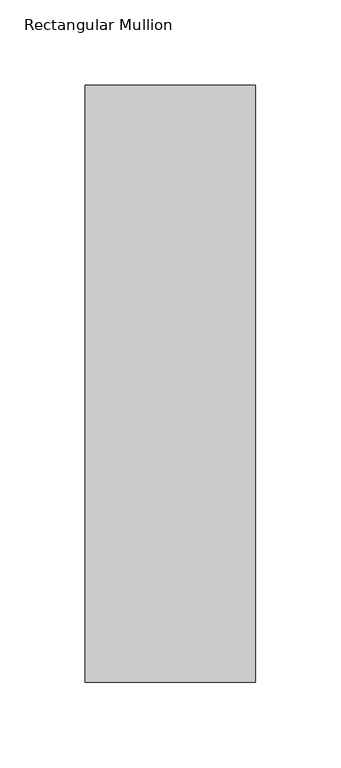
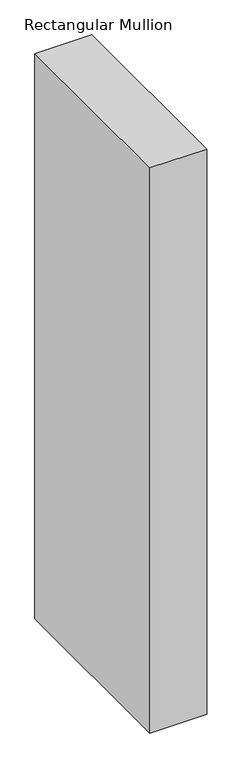
"""IFC4 building model written with IfcOpenShell, lengths in millimetres: member geometry, Rectangular Mullion : WWm-100x350-100mmOffset."""

from ifc_helpers import new_model, si_unit, frame, origin, place, context, project, spatial, polyline, outline, extrude, source, transform, mapped, element, save


def rectangular_mullion_53cec424(model_context):
    return source(origin(), model_context, "Body", "SweptSolid", [
        extrude(outline(polyline([(0.0, 175.0), (0.0, -175.0), (-100.0, -175.0), (-100.0, 175.0), (0.0, 175.0)])), frame((0.0, 0.0, -1050.0), z_axis=(0.0, 0.0, 1.0), x_axis=(1.0, 0.0, 0.0)), (0.0, 0.0, 1.0), 1050.0),
    ])


if __name__ == "__main__":
    model = new_model("IFC4")
    model_context = context("Model", 3, world=origin())
    ifc_project = project(units=[si_unit("LENGTHUNIT", "METRE", prefix="MILLI")], contexts=[model_context])
    site = spatial("IfcSite", under=ifc_project)
    building = spatial("IfcBuilding", under=site)
    placement = place(None, origin())
    rectangular_mullion_shape = rectangular_mullion_53cec424(model_context)
    element("IfcMember", 1, ObjectType="Rectangular Mullion : WWm-100x350-100mmOffset", at=placement, inside=building, context=model_context, shape_type="MappedRepresentation", body=[
        mapped(rectangular_mullion_shape, transform((0.0, 0.0, 0.0), x_axis=(1.0, 0.0, 0.0), y_axis=(0.0, 1.0, 0.0), z_axis=(0.0, 0.0, 1.0))),
    ])
    save(model, "model.ifc")

# Revit data of these elements
# Type "Rectangular Mullion : WWm-100x350-100mmOffset"
#   built-in parameter 1007304 = 1.14829 (stored number, unit not read)
#   built-in parameter 1007301 = 0.164042 (stored number, unit not read)
#   built-in parameter 1007300 = 0.164042 (stored number, unit not read)
# Element 1 (IfcMember, "Rectangular Mullion : WWm-100x350-100mmOffset")
#   Materials on its faces: "WW-EC-RGB-Mullion"
# Materials
#   "WW-EC-RGB-Mullion": class "Generic", colour RGB 255 255 255, transparency 0, Comments = "If region requests black mullions, switch asset color to RGB 25-25-25", Description = "Generic Color", Cost = 0
